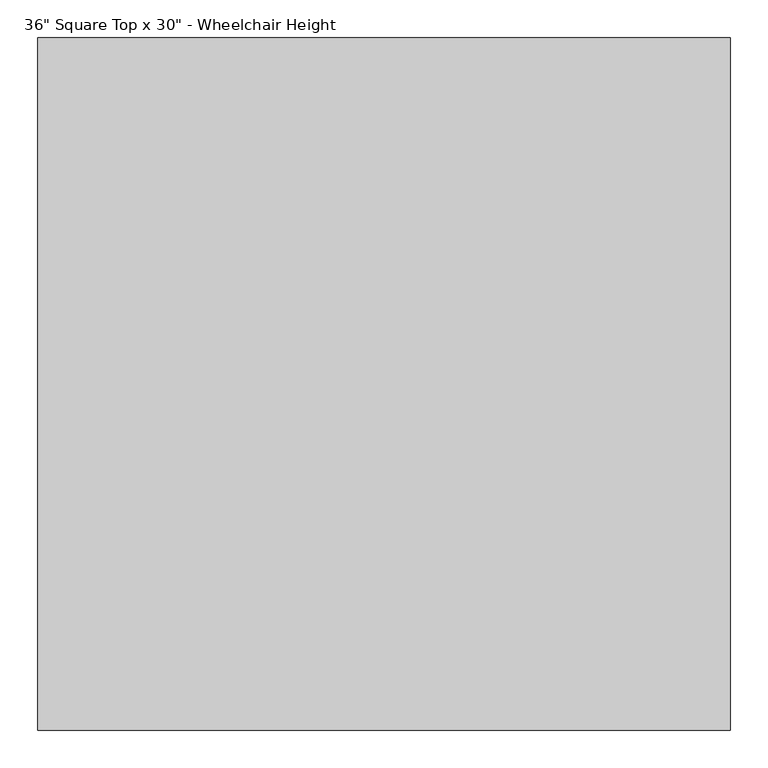
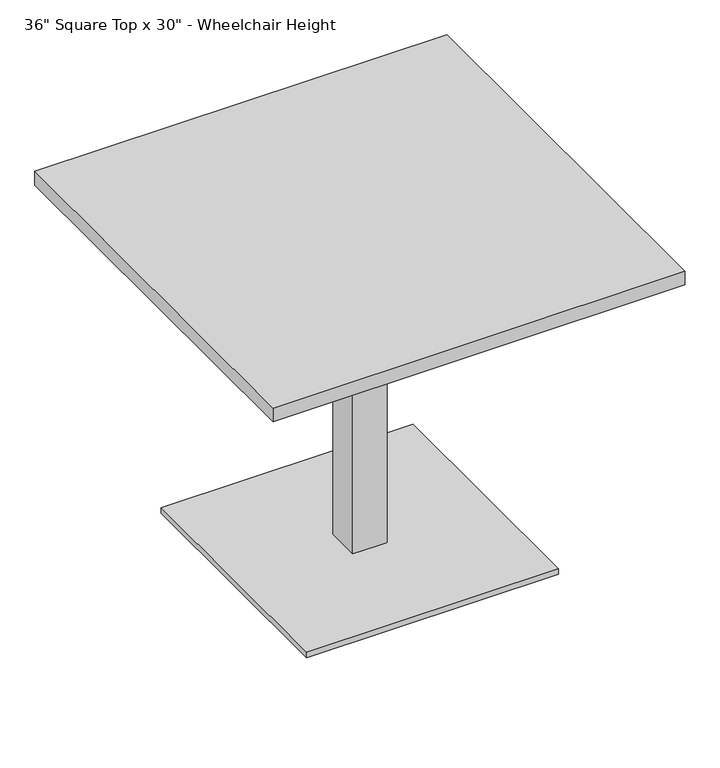
"""IFC4 building model written with IfcOpenShell, lengths in millimetres: furniture geometry."""

from ifc_helpers import new_model, si_unit, point, frame, frame_2d, origin, origin_with_axes, place, context, project, spatial, polyline, circle_curve, trimmed, segment, composite_curve, outline, extrude, source, transform, mapped, element, save


def furniture_8b32ef4e(model_context):
    return source(origin(), model_context, "Body", "SweptSolid", [
        extrude(outline(composite_curve([segment(trimmed(circle_curve(frame_2d((107.7630735, 107.7630735)), 31.75), [point((77.0949285, 99.5455688))], [point((99.5455688, 77.0949285))], False, "CARTESIAN"), True, "CONTINUOUS"), segment(trimmed(circle_curve(frame_2d((97.9020678, 70.9612995)), 6.35), [point((99.5455688, 77.0949285))], [point((93.4119398, 75.4514275))], True, "CARTESIAN"), True, "CONTINUOUS"), segment(polyline([(93.4119398, 75.4514275), (17.9605122, 0.0), (93.4119398, -75.4514275)]), True, "CONTINUOUS"), segment(trimmed(circle_curve(frame_2d((97.9020678, -70.9612995)), 6.35), [point((93.4119398, -75.4514275))], [point((99.5455688, -77.0949285))], True, "CARTESIAN"), True, "CONTINUOUS"), segment(trimmed(circle_curve(frame_2d((107.7630735, -107.7630735)), 31.75), [point((99.5455688, -77.0949285))], [point((77.0949285, -99.5455688))], False, "CARTESIAN"), True, "CONTINUOUS"), segment(trimmed(circle_curve(frame_2d((70.9612995, -97.9020678)), 6.35), [point((77.0949285, -99.5455688))], [point((75.4514275, -93.4119398))], True, "CARTESIAN"), True, "CONTINUOUS"), segment(polyline([(75.4514275, -93.4119398), (0.0, -17.9605122), (-75.4514275, -93.4119398)]), True, "CONTINUOUS"), segment(trimmed(circle_curve(frame_2d((-70.9612995, -97.9020678)), 6.35), [point((-75.4514275, -93.4119398))], [point((-77.0949285, -99.5455688))], True, "CARTESIAN"), True, "CONTINUOUS"), segment(trimmed(circle_curve(frame_2d((-107.7630735, -107.7630735)), 31.75), [point((-77.0949285, -99.5455688))], [point((-99.5455688, -77.0949285))], False, "CARTESIAN"), True, "CONTINUOUS"), segment(trimmed(circle_curve(frame_2d((-97.9020678, -70.9612995)), 6.35), [point((-99.5455688, -77.0949285))], [point((-93.4119398, -75.4514275))], True, "CARTESIAN"), True, "CONTINUOUS"), segment(polyline([(-93.4119398, -75.4514275), (-17.9605122, 0.0), (-93.4119398, 75.4514275)]), True, "CONTINUOUS"), segment(trimmed(circle_curve(frame_2d((-97.9020678, 70.9612995)), 6.35), [point((-93.4119398, 75.4514275))], [point((-99.5455688, 77.0949285))], True, "CARTESIAN"), True, "CONTINUOUS"), segment(trimmed(circle_curve(frame_2d((-107.7630735, 107.7630735)), 31.75), [point((-99.5455688, 77.0949285))], [point((-77.0949285, 99.5455688))], False, "CARTESIAN"), True, "CONTINUOUS"), segment(trimmed(circle_curve(frame_2d((-70.9612995, 97.9020678)), 6.35), [point((-77.0949285, 99.5455688))], [point((-75.4514275, 93.4119398))], True, "CARTESIAN"), True, "CONTINUOUS"), segment(polyline([(-75.4514275, 93.4119398), (0.0, 17.9605122), (75.4514275, 93.4119398)]), True, "CONTINUOUS"), segment(trimmed(circle_curve(frame_2d((70.9612995, 97.9020678)), 6.35), [point((75.4514275, 93.4119398))], [point((77.0949285, 99.5455688))], True, "CARTESIAN"), True, "CONTINUOUS")], self_intersect=False)), frame((0.0, 0.0, 723.9), z_axis=(0.0, 0.0, 1.0), x_axis=(1.0, 0.0, 0.0)), (0.0, 0.0, 1.0), 6.35),
        extrude(outline(polyline([(-38.1, 38.1), (38.1, 38.1), (38.1, -38.1), (-38.1, -38.1), (-38.1, 38.1)])), frame((0.0, 0.0, 19.05), z_axis=(0.0, 0.0, 1.0), x_axis=(1.0, 0.0, 0.0)), (0.0, 0.0, 1.0), 704.85),
        extrude(outline(composite_curve([segment(trimmed(circle_curve(frame_2d((-251.0506403, -251.0506403)), 12.7), [point((-263.7506403, -251.0506403))], [point((-238.3506403, -251.0506403))], False, "CARTESIAN"), True, "CONTINUOUS"), segment(trimmed(circle_curve(frame_2d((-251.0506403, -251.0506403)), 12.7), [point((-238.3506403, -251.0506403))], [point((-263.7506403, -251.0506403))], False, "CARTESIAN"), True, "CONTINUOUS")], self_intersect=False)), origin_with_axes(), (0.0, 0.0, 1.0), 6.35),
        extrude(outline(composite_curve([segment(trimmed(circle_curve(frame_2d((-251.0506403, 251.0506403)), 12.7), [point((-263.7506403, 251.0506403))], [point((-238.3506403, 251.0506403))], False, "CARTESIAN"), True, "CONTINUOUS"), segment(trimmed(circle_curve(frame_2d((-251.0506403, 251.0506403)), 12.7), [point((-238.3506403, 251.0506403))], [point((-263.7506403, 251.0506403))], False, "CARTESIAN"), True, "CONTINUOUS")], self_intersect=False)), origin_with_axes(), (0.0, 0.0, 1.0), 6.35),
        extrude(outline(composite_curve([segment(trimmed(circle_curve(frame_2d((251.0506403, -251.0506403)), 12.7), [point((238.3506403, -251.0506403))], [point((263.7506403, -251.0506403))], False, "CARTESIAN"), True, "CONTINUOUS"), segment(trimmed(circle_curve(frame_2d((251.0506403, -251.0506403)), 12.7), [point((263.7506403, -251.0506403))], [point((238.3506403, -251.0506403))], False, "CARTESIAN"), True, "CONTINUOUS")], self_intersect=False)), origin_with_axes(), (0.0, 0.0, 1.0), 6.35),
        extrude(outline(composite_curve([segment(trimmed(circle_curve(frame_2d((251.0506403, 251.0506403)), 12.7), [point((238.3506403, 251.0506403))], [point((263.7506403, 251.0506403))], False, "CARTESIAN"), True, "CONTINUOUS"), segment(trimmed(circle_curve(frame_2d((251.0506403, 251.0506403)), 12.7), [point((263.7506403, 251.0506403))], [point((238.3506403, 251.0506403))], False, "CARTESIAN"), True, "CONTINUOUS")], self_intersect=False)), origin_with_axes(), (0.0, 0.0, 1.0), 6.35),
        extrude(outline(polyline([(279.4, 279.4), (279.4, -279.4), (-279.4, -279.4), (-279.4, 279.4), (279.4, 279.4)])), frame((0.0, 0.0, 6.35), z_axis=(0.0, 0.0, 1.0), x_axis=(1.0, 0.0, 0.0)), (0.0, 0.0, 1.0), 12.7),
        extrude(outline(polyline([(457.2, 457.2), (457.2, -457.2), (-457.2, -457.2), (-457.2, 457.2), (457.2, 457.2)])), frame((0.0, 0.0, 730.25), z_axis=(0.0, 0.0, 1.0), x_axis=(1.0, 0.0, 0.0)), (0.0, 0.0, 1.0), 31.75),
    ])


if __name__ == "__main__":
    model = new_model("IFC4")
    model_context = context("Model", 3, world=origin())
    ifc_project = project(units=[si_unit("LENGTHUNIT", "METRE", prefix="MILLI")], contexts=[model_context])
    site = spatial("IfcSite", under=ifc_project)
    building = spatial("IfcBuilding", under=site)
    placement = place(None, origin())
    furniture_shape = furniture_8b32ef4e(model_context)
    element("IfcFurniture", 1, ObjectType="Falcon 7700 Series Pedestal Base : 36\" Square Top x 30\" - Wheelchair Height", at=placement, inside=building, context=model_context, shape_type="MappedRepresentation", body=[
        mapped(furniture_shape, transform((0.0, 0.0, 0.0), x_axis=(1.0, 0.0, 0.0), y_axis=(0.0, 1.0, 0.0), z_axis=(0.0, 0.0, 1.0))),
    ])
    save(model, "model.ifc")

# Revit data of these elements
# Type "Falcon 7700 Series Pedestal Base : 36\" Square Top x 30\" - Wheelchair Height"
#   URL = "http://www.commercialfurnituregroup.com/"
#   Product URL = "http://www.falconproducts.com/product/10525/Square-Table-Base.html"
#   Modeled By [instance default] = "http://www.therevitcollection.com"
#   Model Line = "Table Bases"
#   Model = "7700 Series"
#   Description = "Single Pedestal Table Base"
#   Brand = "Falcon"
#   Manufacturer = "Commercial Furniture Group Inc."
#   Assembly Code = "E2020200"
#   Table Width = 3' - 0"
#   Table Depth = 3' - 0"
#   Radius = 1' - 6"
#   Base Width = 1' - 10"
#   Table Thickness [instance default] = 0' - 1 1/4"
#   Height = 2' - 6"
#   Base Depth = 1' - 10"
#   Roundtop = no
#   RectangleTop = yes
#   Tabletop [instance default] = none
#   Table Base [instance default] = none
#   Type Comments = ""
#   Default Elevation = 0
# Element 1 (IfcFurniture, "Falcon 7700 Series Pedestal Base : 36\" Square Top x 30\" - Wheelchair Height")
#   Tabletop = Metal - Aluminum
#   Table Base = Metal - Aluminum
#   Materials on its faces: "Metal - Aluminum"
# Materials
#   "Metal - Aluminum": class "Metal", colour RGB 247 247 247, transparency 0
